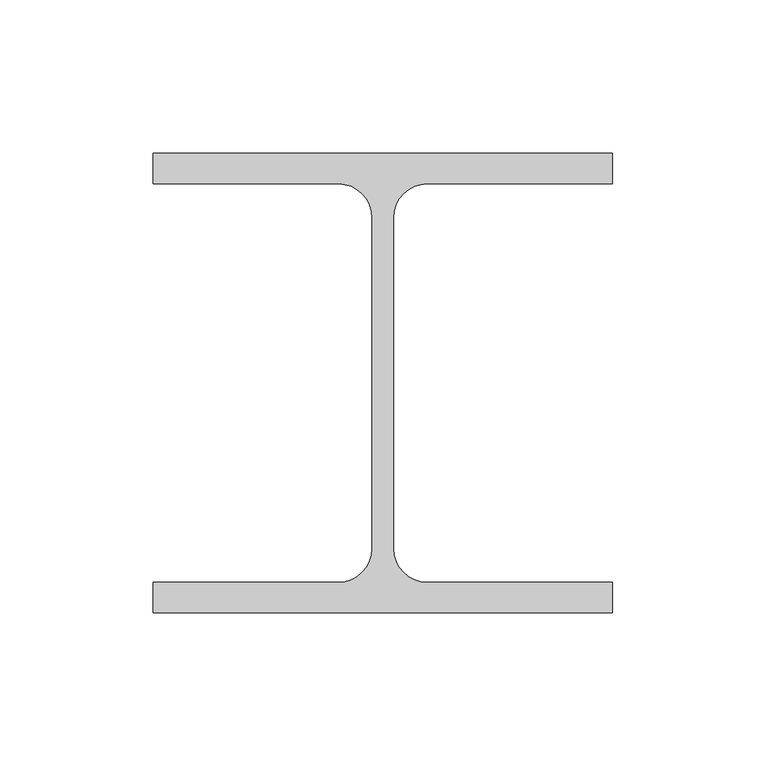
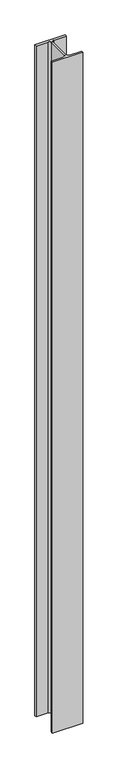
"""IFC4 building model written with IfcOpenShell, lengths in millimetres: column geometry, 0912_Steel Column_H_KSD3502 : H_SC_ASC_H-150x150x7x10."""

import ifcopenshell
import ifcopenshell.guid

model = None  # the IFC model being written
_history = None  # IfcOwnerHistory: only IFC2X3 demands one
_inside = {}  # id of a spatial element -> (the spatial element, [elements in it])
_under = {}  # id of a project, library or spatial element -> (it, [spatial elements below it])
_declared = {}  # id of a project -> (the project, [libraries it declares])
_typed = {}  # id of a type object -> (the type object, [elements of that type])
_made_of = {}  # id of a material, layer set ... -> (it, [elements and type objects made of it])


def new_model(schema):
    """Start an empty IFC model of exactly this schema.

    Asked for "IFC4X3", IfcOpenShell would pick the latest addendum, in which some entities
    have other attributes; the version numbers below select the first issue.
    IFC2X3 requires an IfcOwnerHistory on every rooted entity: one is made here for all.
    """
    global model, _history
    if schema == "IFC4X3":
        model = ifcopenshell.file(schema_version=(4, 3, 0, 0))
    else:
        model = ifcopenshell.file(schema=schema)
    _inside.clear()
    _under.clear()
    _declared.clear()
    _typed.clear()
    _made_of.clear()
    _history = None
    if model.schema == "IFC2X3":
        org = make("IfcOrganization", Name="unknown")
        user = make(
            "IfcPersonAndOrganization",
            ThePerson=make("IfcPerson", FamilyName="unknown"),
            TheOrganization=org,
        )
        app = make(
            "IfcApplication",
            ApplicationDeveloper=org,
            Version="unknown",
            ApplicationFullName="unknown",
            ApplicationIdentifier="unknown",
        )
        _history = make(
            "IfcOwnerHistory",
            OwningUser=user,
            OwningApplication=app,
            ChangeAction="ADDED",
            CreationDate=0,
        )
    return model


def make(cls, **values):
    """One entity of the class cls with the attributes given. An attribute that is None is left unset."""
    return model.create_entity(
        cls, **{name: value for name, value in values.items() if value is not None}
    )


def rooted(cls, **values):
    """An entity with a GlobalId (a new one), such as an element, a storey or a relation."""
    return make(cls, GlobalId=ifcopenshell.guid.new(), OwnerHistory=_history, **values)


def si_unit(unit_type, name, prefix=None):
    """IfcSIUnit, for example si_unit("LENGTHUNIT", "METRE", prefix="MILLI")."""
    return make("IfcSIUnit", UnitType=unit_type, Prefix=prefix, Name=name)


def assignment(units):
    """IfcUnitAssignment: the units of a project."""
    return None if units is None else make("IfcUnitAssignment", Units=units)


def point(xyz):
    """IfcCartesianPoint."""
    return None if xyz is None else make("IfcCartesianPoint", Coordinates=xyz)


def direction(xyz):
    """IfcDirection."""
    return None if xyz is None else make("IfcDirection", DirectionRatios=xyz)


def frame(location, z_axis=None, x_axis=None):
    """IfcAxis2Placement3D, a coordinate frame: its origin and axes. An axis left out is left unset."""
    return make(
        "IfcAxis2Placement3D",
        Location=point(location),
        Axis=direction(z_axis),
        RefDirection=direction(x_axis),
    )


def frame_2d(location, x_axis=None):
    """IfcAxis2Placement2D, a coordinate frame in the plane: its origin and x axis."""
    return make(
        "IfcAxis2Placement2D", Location=point(location), RefDirection=direction(x_axis)
    )


def origin():
    """The frame at (0, 0, 0) with its axes left unset."""
    return frame((0.0, 0.0, 0.0))


def place(relative_to, where):
    """IfcLocalPlacement: puts the frame where relative to a parent placement (None: the world)."""
    return make(
        "IfcLocalPlacement", PlacementRelTo=relative_to, RelativePlacement=where
    )


def context(
    kind, dimensions, precision=None, world=None, true_north=None, identifier=None
):
    """IfcGeometricRepresentationContext, for example the 3D "Model" context."""
    return make(
        "IfcGeometricRepresentationContext",
        ContextIdentifier=identifier,
        ContextType=kind,
        CoordinateSpaceDimension=dimensions,
        Precision=precision,
        WorldCoordinateSystem=world,
        TrueNorth=true_north,
    )


def project(units=None, contexts=None):
    """IfcProject with its units and contexts."""
    return rooted(
        "IfcProject",
        Name="project",
        RepresentationContexts=contexts,
        UnitsInContext=assignment(units),
    )


def spatial(cls, under=None, at=None, **own):
    """A site, building, storey or space (cls), placed at a placement, below another one or the project."""
    s = rooted(cls, ObjectPlacement=at, **own)
    if under is not None:
        _under.setdefault(under.id(), (under, []))[1].append(s)
    return s


def polyline(points):
    """IfcPolyline through the points."""
    return make("IfcPolyline", Points=[point(p) for p in points])


def circle_curve(where, radius):
    """IfcCircle in the frame where."""
    return make("IfcCircle", Position=where, Radius=radius)


def trimmed(basis, trim1, trim2, sense, master):
    """IfcTrimmedCurve: the piece of a basis curve between two trims."""
    return make(
        "IfcTrimmedCurve",
        BasisCurve=basis,
        Trim1=trim1,
        Trim2=trim2,
        SenseAgreement=sense,
        MasterRepresentation=master,
    )


def segment(curve, same_sense, transition):
    """IfcCompositeCurveSegment."""
    return make(
        "IfcCompositeCurveSegment",
        Transition=transition,
        SameSense=same_sense,
        ParentCurve=curve,
    )


def composite_curve(segments, self_intersect=None):
    """IfcCompositeCurve: segments joined end to end."""
    return make("IfcCompositeCurve", Segments=segments, SelfIntersect=self_intersect)


def outline(outer, holes=None, kind="AREA"):
    """IfcArbitraryClosedProfileDef: a profile drawn as a closed curve; with holes, ...WithVoids."""
    if holes is None:
        return make("IfcArbitraryClosedProfileDef", ProfileType=kind, OuterCurve=outer)
    return make(
        "IfcArbitraryProfileDefWithVoids",
        ProfileType=kind,
        OuterCurve=outer,
        InnerCurves=holes,
    )


def extrude(swept, where, along, depth):
    """IfcExtrudedAreaSolid: the profile swept, set in the frame where, extruded along a direction by depth."""
    return make(
        "IfcExtrudedAreaSolid",
        SweptArea=swept,
        Position=where,
        ExtrudedDirection=direction(along),
        Depth=depth,
    )


def shape(context_of_items, identifier, shape_type, items):
    """IfcShapeRepresentation: the items that make up one representation, for example the "Body"."""
    return make(
        "IfcShapeRepresentation",
        ContextOfItems=context_of_items,
        RepresentationIdentifier=identifier,
        RepresentationType=shape_type,
        Items=items,
    )


def source(mapping_origin, context_of_items, identifier, shape_type, items):
    """IfcRepresentationMap: a shape defined once, which mapped items show again and again."""
    return make(
        "IfcRepresentationMap",
        MappingOrigin=mapping_origin,
        MappedRepresentation=shape(context_of_items, identifier, shape_type, items),
    )


def transform(
    local_origin,
    x_axis=None,
    y_axis=None,
    z_axis=None,
    scale=None,
    scale2=None,
    scale3=None,
    uniform=True,
):
    """IfcCartesianTransformationOperator3D, or its non-uniform kind. x_axis, y_axis, z_axis: its Axis1, 2, 3."""
    if uniform:
        return make(
            "IfcCartesianTransformationOperator3D",
            Axis1=direction(x_axis),
            Axis2=direction(y_axis),
            LocalOrigin=point(local_origin),
            Scale=scale,
            Axis3=direction(z_axis),
        )
    return make(
        "IfcCartesianTransformationOperator3DnonUniform",
        Axis1=direction(x_axis),
        Axis2=direction(y_axis),
        LocalOrigin=point(local_origin),
        Scale=scale,
        Axis3=direction(z_axis),
        Scale2=scale2,
        Scale3=scale3,
    )


def mapped(mapping_source, mapping_target):
    """IfcMappedItem: shows the shape of a source again, moved by a transform."""
    return make(
        "IfcMappedItem", MappingSource=mapping_source, MappingTarget=mapping_target
    )


def made_of(thing, what):
    """Note that an element or type object is made of a material, layer set ...; save() writes the relation."""
    if what is not None:
        _made_of.setdefault(what.id(), (what, []))[1].append(thing)
    return thing


def element(
    cls,
    number,
    at=None,
    inside=None,
    cuts=None,
    type_object=None,
    material=None,
    context=None,
    identifier="Body",
    shape_type=None,
    held_by="IfcProductDefinitionShape",
    body=None,
    shapes=None,
    **own,
):
    """One element of the class cls, such as IfcWall. Its Tag is "e" and its number.

    at: its placement. inside: the storey or other place that contains it. cuts: it is an
    opening in that element (IfcRelVoidsElement). A single representation is given by context,
    identifier, shape_type and body (its items); several are given by shapes. held_by: the class
    of the entity that holds the representations. save() writes the other relations.
    """
    e = rooted(cls, Tag="e%d" % number, ObjectPlacement=at, **own)
    if body is not None:
        shapes = [shape(context, identifier, shape_type, body)]
    if shapes is not None:
        e.Representation = make(held_by, Representations=shapes)
    if inside is not None:
        _inside.setdefault(inside.id(), (inside, []))[1].append(e)
    if cuts is not None:
        rooted(
            "IfcRelVoidsElement", RelatingBuildingElement=cuts, RelatedOpeningElement=e
        )
    if type_object is not None:
        _typed.setdefault(type_object.id(), (type_object, []))[1].append(e)
    return made_of(e, material)


def aggregate(whole, parts):
    """IfcRelAggregates: a whole, such as a stair, and the parts it consists of."""
    return rooted("IfcRelAggregates", RelatingObject=whole, RelatedObjects=parts)


def save(model, path):
    """Write the relations noted so far, then the file.

    IfcRelAggregates (storeys below a building ...), IfcRelContainedInSpatialStructure (elements
    in a storey), IfcRelDefinesByType, IfcRelAssociatesMaterial and IfcRelDeclares: one each for
    every whole, place, type object, material and project.
    """
    for whole, parts in _under.values():
        aggregate(whole, parts)
    for where, things in _inside.values():
        rooted(
            "IfcRelContainedInSpatialStructure",
            RelatedElements=things,
            RelatingStructure=where,
        )
    for kind, things in _typed.values():
        rooted("IfcRelDefinesByType", RelatedObjects=things, RelatingType=kind)
    for what, things in _made_of.values():
        rooted("IfcRelAssociatesMaterial", RelatedObjects=things, RelatingMaterial=what)
    for by, libraries in _declared.values():
        rooted("IfcRelDeclares", RelatingContext=by, RelatedDefinitions=libraries)
    model.write(path)


def column_e739ab66(model_context):
    return source(origin(), model_context, "Body", "SweptSolid", [
        extrude(outline(composite_curve([segment(polyline([(75.0, 75.0), (75.0, 65.0), (14.5, 65.0)]), True, "CONTINUOUS"), segment(trimmed(circle_curve(frame_2d((14.5, 54.0)), 11.0), [point((14.5, 65.0))], [point((3.5, 54.0))], True, "CARTESIAN"), True, "CONTINUOUS"), segment(polyline([(3.5, 54.0), (3.5, -54.0)]), True, "CONTINUOUS"), segment(trimmed(circle_curve(frame_2d((14.5, -54.0)), 11.0), [point((3.5, -54.0))], [point((14.5, -65.0))], True, "CARTESIAN"), True, "CONTINUOUS"), segment(polyline([(14.5, -65.0), (75.0, -65.0), (75.0, -75.0), (-75.0, -75.0), (-75.0, -65.0), (-14.5, -65.0)]), True, "CONTINUOUS"), segment(trimmed(circle_curve(frame_2d((-14.5, -54.0)), 11.0), [point((-14.5, -65.0))], [point((-3.5, -54.0))], True, "CARTESIAN"), True, "CONTINUOUS"), segment(polyline([(-3.5, -54.0), (-3.5, 54.0)]), True, "CONTINUOUS"), segment(trimmed(circle_curve(frame_2d((-14.5, 54.0)), 11.0), [point((-3.5, 54.0))], [point((-14.5, 65.0))], True, "CARTESIAN"), True, "CONTINUOUS"), segment(polyline([(-14.5, 65.0), (-75.0, 65.0), (-75.0, 75.0), (75.0, 75.0)]), True, "CONTINUOUS")], self_intersect=False)), frame((0.0, 0.0, 599.9720055), z_axis=(0.0, 0.0, 1.0), x_axis=(1.0, 0.0, 0.0)), (0.0, 0.0, 1.0), 3510.0),
    ])


if __name__ == "__main__":
    model = new_model("IFC4")
    model_context = context("Model", 3, world=origin())
    ifc_project = project(units=[si_unit("LENGTHUNIT", "METRE", prefix="MILLI")], contexts=[model_context])
    site = spatial("IfcSite", under=ifc_project)
    building = spatial("IfcBuilding", under=site)
    placement = place(None, origin())
    column_shape = column_e739ab66(model_context)
    element("IfcColumn", 1, ObjectType="0912_Steel Column_H_KSD3502 : H_SC_ASC_H-150x150x7x10", at=placement, inside=building, context=model_context, shape_type="MappedRepresentation", body=[
        mapped(column_shape, transform((0.0, 0.0, 0.0), x_axis=(1.0, 0.0, 0.0), y_axis=(0.0, 1.0, 0.0), z_axis=(0.0, 0.0, 1.0))),
    ])
    save(model, "model.ifc")

# Revit data of these elements
# Type "0912_Steel Column_H_KSD3502 : H_SC_ASC_H-150x150x7x10"
#   H_WM Code_1 = "S01AA002-00001 | Main Steel Structure Fabrication Work | Shelter/Building | Medium Steel - Standard (90KG/M>Weight≥30KG/M) | Material: (   )"
#   H_WM Code_2 = "S03AA028-00001 | Main Steel Structure Erection Work | Shelter/Building | Medium Steel (90KG/M>Weight≥30KG/M) | Material: (   )"
#   H_WM Code_3 = "S01AA010-00001 | Main Steel Structure Fabrication Work | Shelter/Building | Steel Painting/Coating | for Non-Fireproofed Steel Surface, Surface Preparation, Primer, Second & Final Coat | Material: (   )"
#   H_Q'ty Cal Type Tag = "SC-Q2"
#   Width = 15.0 cm
#   Web Thickness = 0.7 cm
#   Web Fillet = 1.1 cm
#   Warping Constant = 27562.5 cm⁶
#   Torsional Moment of Inertia = 11.6007 cm⁴
#   Section Area = 40.14 cm²
#   Plastic Modulus weak axis = 115.0 cm³
#   Plastic Modulus strong axis = 246.0 cm³
#   Perimeter = 0.87 m²/m
#   Nominal Weight = 31.50 kgf/m
#   Moment of Inertia weak axis = 563.00 cm⁴
#   Moment of Inertia strong axis = 1640.00 cm⁴
#   Height = 15.0 cm
#   Flange Thickness = 1.0 cm
#   Elastic Modulus weak axis = 75.1 cm³
#   Elastic Modulus strong axis = 219.0 cm³
#   Centroid Vertical = 7.5 cm
#   Centroid Horizontal = 7.5 cm
#   Structural Material [instance default] = Steel, 45-345
#   Section Name Key = ""
#   Bolt Spacing = 0
#   Assembly Code = ""
# Element 1 (IfcColumn, "0912_Steel Column_H_KSD3502 : H_SC_ASC_H-150x150x7x10")
#   Structural Material = A03AD029-00005_Anchor Bolt (Installation only)_M24
#   Materials on its faces: "A03AD029-00005_Anchor Bolt (Installation only)_M24"
# Materials
#   "Steel, 45-345": class "Metal", colour RGB 189 187 185, transparency 0, Description = "Steel 345 MPa", Cost = 0
#   "A03AD029-00005_Anchor Bolt (Installation only)_M24": class "Unassigned", colour RGB 84 83 81, transparency 0, Cost = 0
